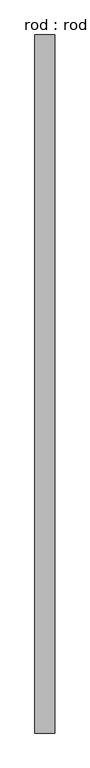
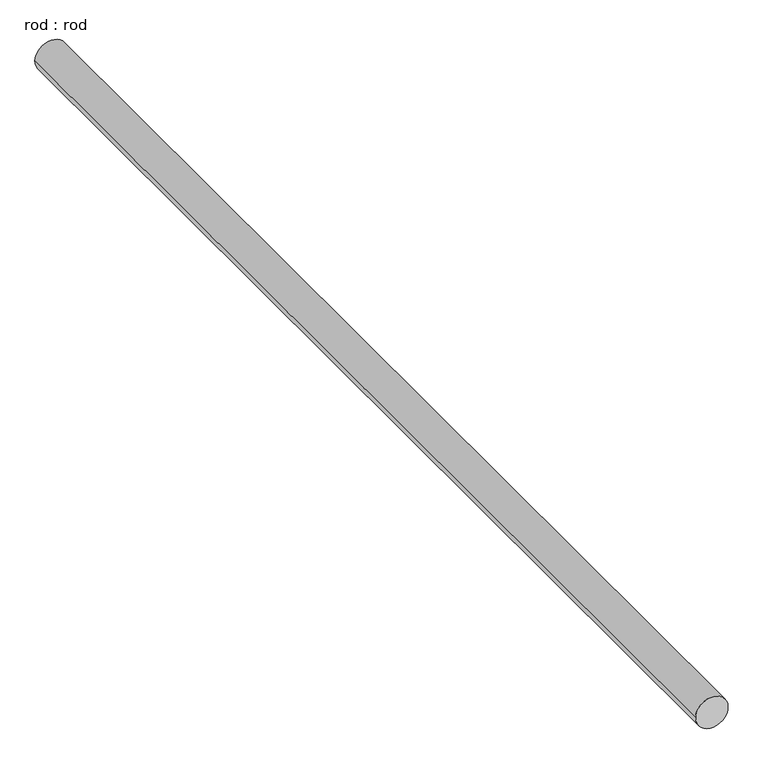
"""IFC4 building model written with IfcOpenShell, lengths in millimetres: proxy geometry, rod : rod."""

from ifc_helpers import new_model, si_unit, point, frame, frame_2d, origin, place, context, project, spatial, circle_curve, trimmed, segment, composite_curve, outline, extrude, source, transform, mapped, element, save


def rod_rod_ba611c6c(model_context):
    return source(origin(), model_context, "Body", "SweptSolid", [
        extrude(outline(composite_curve([segment(trimmed(circle_curve(frame_2d((0.0108462, 0.0)), 200.0), [point((0.0108462, 200.0))], [point((0.0108462, -200.0))], False, "CARTESIAN"), True, "CONTINUOUS"), segment(trimmed(circle_curve(frame_2d((0.0108462, 0.0)), 200.0), [point((0.0108462, -200.0))], [point((0.0108462, 200.0))], False, "CARTESIAN"), True, "CONTINUOUS")], self_intersect=False)), frame((0.0, -2969.7713847, 0.0), z_axis=(0.0, 1.0, 0.0), x_axis=(0.0, 0.0, 1.0)), (0.0, 0.0, 1.0), 14125.0),
    ])


if __name__ == "__main__":
    model = new_model("IFC4")
    model_context = context("Model", 3, world=origin())
    ifc_project = project(units=[si_unit("LENGTHUNIT", "METRE", prefix="MILLI")], contexts=[model_context])
    site = spatial("IfcSite", under=ifc_project)
    building = spatial("IfcBuilding", under=site)
    placement = place(None, origin())
    rod_rod_shape = rod_rod_ba611c6c(model_context)
    element("IfcBuildingElementProxy", 1, Name="rod : rod", ObjectType="rod : rod", at=placement, inside=building, context=model_context, shape_type="MappedRepresentation", body=[
        mapped(rod_rod_shape, transform((0.0, 0.0, 0.0), x_axis=(1.0, 0.0, 0.0), y_axis=(0.0, 1.0, 0.0), z_axis=(0.0, 0.0, 1.0))),
    ])
    save(model, "model.ifc")

# Revit data of these elements
# Type "rod : rod"
#   Default Elevation = 0
